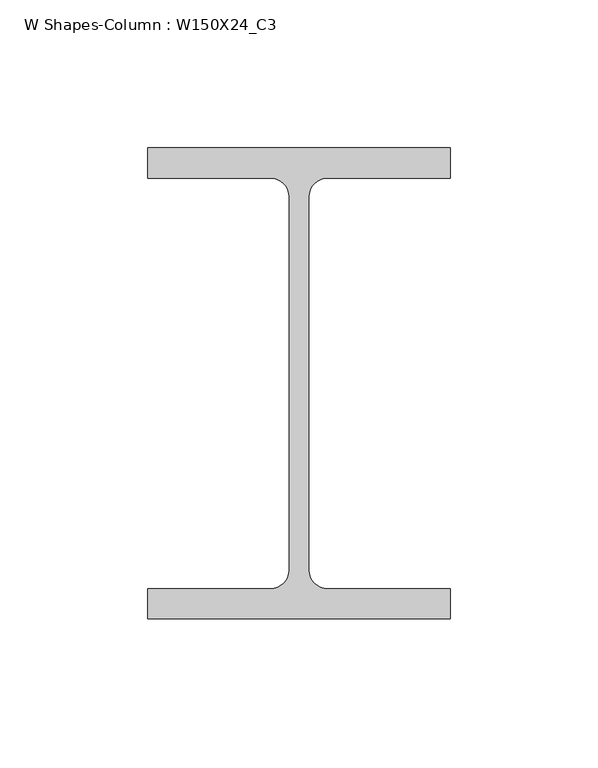
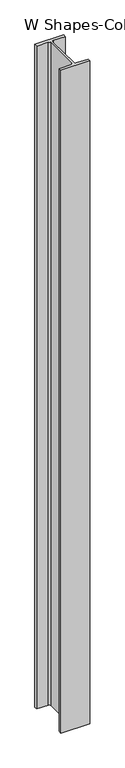
"""IFC4 building model written with IfcOpenShell, lengths in millimetres: column geometry, W Shapes-Column : W150X24_C3."""

from ifc_helpers import new_model, si_unit, point, frame, frame_2d, origin, place, context, project, spatial, polyline, circle_curve, trimmed, segment, composite_curve, outline, extrude, source, transform, mapped, element, save


def w_shapes_column_w150x24_c3_0915dd23(model_context):
    return source(origin(), model_context, "Body", "SweptSolid", [
        extrude(outline(composite_curve([segment(polyline([(51.181, 79.756), (51.181, 69.469), (9.652, 69.469)]), True, "CONTINUOUS"), segment(trimmed(circle_curve(frame_2d((9.652, 63.119)), 6.35), [point((9.652, 69.469))], [point((3.302, 63.119))], True, "CARTESIAN"), True, "CONTINUOUS"), segment(polyline([(3.302, 63.119), (3.302, -63.119)]), True, "CONTINUOUS"), segment(trimmed(circle_curve(frame_2d((9.652, -63.119)), 6.35), [point((3.302, -63.119))], [point((9.652, -69.469))], True, "CARTESIAN"), True, "CONTINUOUS"), segment(polyline([(9.652, -69.469), (51.181, -69.469), (51.181, -79.756), (-51.181, -79.756), (-51.181, -69.469), (-9.652, -69.469)]), True, "CONTINUOUS"), segment(trimmed(circle_curve(frame_2d((-9.652, -63.119)), 6.35), [point((-9.652, -69.469))], [point((-3.302, -63.119))], True, "CARTESIAN"), True, "CONTINUOUS"), segment(polyline([(-3.302, -63.119), (-3.302, 63.119)]), True, "CONTINUOUS"), segment(trimmed(circle_curve(frame_2d((-9.652, 63.119)), 6.35), [point((-3.302, 63.119))], [point((-9.652, 69.469))], True, "CARTESIAN"), True, "CONTINUOUS"), segment(polyline([(-9.652, 69.469), (-51.181, 69.469), (-51.181, 79.756), (51.181, 79.756)]), True, "CONTINUOUS")], self_intersect=False)), frame((0.0, 0.0, 3526.0), z_axis=(0.0, 0.0, 1.0), x_axis=(1.0, 0.0, 0.0)), (0.0, 0.0, 1.0), 2484.0),
    ])


if __name__ == "__main__":
    model = new_model("IFC4")
    model_context = context("Model", 3, world=origin())
    ifc_project = project(units=[si_unit("LENGTHUNIT", "METRE", prefix="MILLI")], contexts=[model_context])
    site = spatial("IfcSite", under=ifc_project)
    building = spatial("IfcBuilding", under=site)
    placement = place(None, origin())
    w_shapes_column_w150x24_c3_shape = w_shapes_column_w150x24_c3_0915dd23(model_context)
    element("IfcColumn", 1, ObjectType="W Shapes-Column : W150X24_C3", at=placement, inside=building, context=model_context, shape_type="MappedRepresentation", body=[
        mapped(w_shapes_column_w150x24_c3_shape, transform((0.0, 0.0, 0.0), x_axis=(1.0, 0.0, 0.0), y_axis=(0.0, 1.0, 0.0), z_axis=(0.0, 0.0, 1.0))),
    ])
    save(model, "model.ifc")

# Revit data of these elements
# Type "W Shapes-Column : W150X24_C3"
#   Section Name Key = "W6x16"
#   Assembly Code = "B10"
#   Width = 10.2362 cm
#   Web Thickness = 0.6604 cm
#   Web Fillet = 0.635 cm
#   Warping Constant = 10258.1 cm⁶
#   Torsional Moment of Inertia = 9.28196 cm⁴
#   Section Area = 30.5806 cm²
#   Plastic Modulus weak axis = 55.5521 cm³
#   Plastic Modulus strong axis = 191.729 cm³
#   Perimeter = 0.704088 m²/m
#   Nominal Weight = 23.8106 kgf/m
#   Moment of Inertia weak axis = 184.391 cm⁴
#   Moment of Inertia strong axis = 1336.10 cm⁴
#   Height = 15.9512 cm
#   Flange Thickness = 1.0287 cm
#   Elastic Modulus weak axis = 36.0515 cm³
#   Elastic Modulus strong axis = 167.148 cm³
#   Clear Web Height = 19.05 cm
#   Centroid Vertical = 7.9756 cm
#   Centroid Horizontal = 5.1181 cm
#   Bolt Spacing = 5.715 cm
#   Structural Material [instance default] = Steel ASTM A992
#   Principal Axes Angle = 0
# Element 1 (IfcColumn, "W Shapes-Column : W150X24_C3")
#   Structural Material = none
# Materials
#   "Steel ASTM A992": class "Metal", colour RGB 199 199 199, transparency 0, Description = "Structural steel 50ksi", Cost = 0
